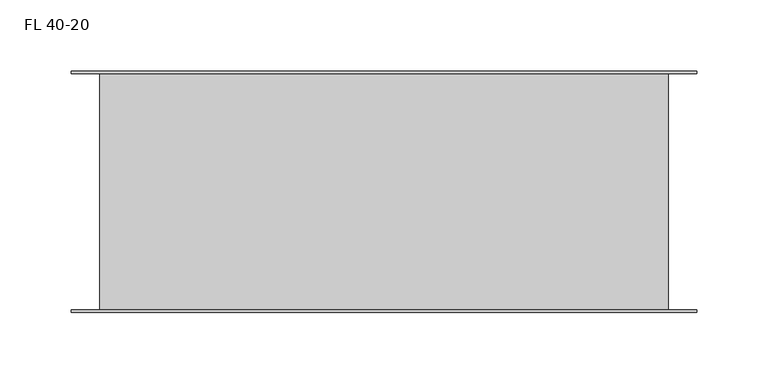
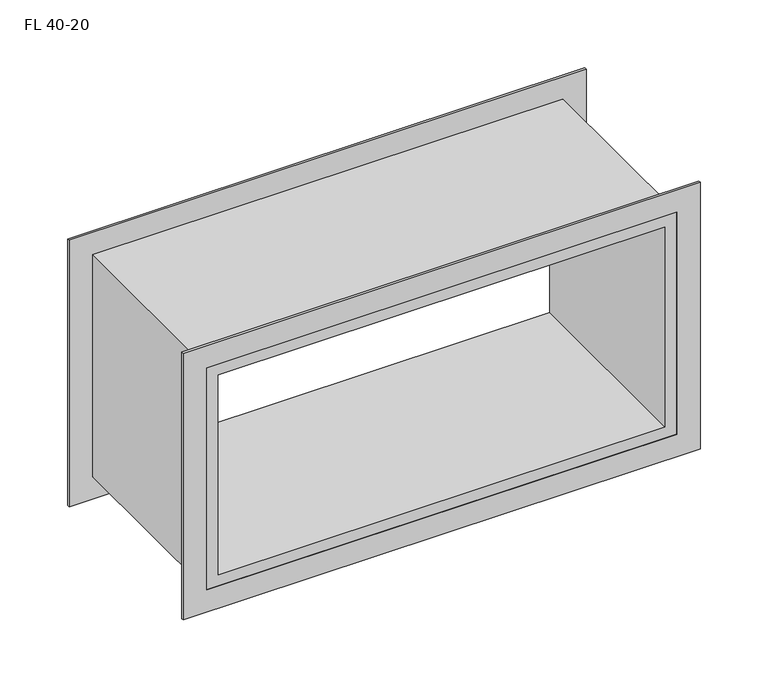
"""IFC4 building model written with IfcOpenShell, lengths in millimetres: proxy geometry, Обратный клапан FL : FL 40-20."""

from ifc_helpers import new_model, si_unit, frame, origin, place, context, project, spatial, polyline, outline, extrude, source, transform, mapped, element, save


def fl_40_20_b5c6f90e(model_context):
    return source(origin(), model_context, "Body", "SweptSolid", [
        extrude(outline(polyline([(120.0, 220.0), (120.0, -220.0), (-120.0, -220.0), (-120.0, 220.0), (120.0, 220.0)]), holes=[polyline([(-100.0, 200.0), (-100.0, -200.0), (100.0, -200.0), (100.0, 200.0), (-100.0, 200.0)])]), frame((0.0, 83.0, 0.0), z_axis=(0.0, 1.0, 0.0), x_axis=(0.0, 0.0, 1.0)), (0.0, 0.0, 1.0), 2.0),
        extrude(outline(polyline([(120.0, -220.0), (-120.0, -220.0), (-120.0, 220.0), (120.0, 220.0), (120.0, -220.0)]), holes=[polyline([(100.0, 200.0), (-100.0, 200.0), (-100.0, -200.0), (100.0, -200.0), (100.0, 200.0)])]), frame((0.0, -85.0, 0.0), z_axis=(0.0, 1.0, 0.0), x_axis=(0.0, 0.0, 1.0)), (0.0, 0.0, 1.0), 2.0),
        extrude(outline(polyline([(100.0, 200.0), (100.0, -200.0), (-100.0, -200.0), (-100.0, 200.0), (100.0, 200.0)]), holes=[polyline([(90.0, 190.0), (-90.0, 190.0), (-90.0, -190.0), (90.0, -190.0), (90.0, 190.0)])]), frame((0.0, -85.0, 0.0), z_axis=(0.0, 1.0, 0.0), x_axis=(0.0, 0.0, 1.0)), (0.0, 0.0, 1.0), 170.0),
    ])


if __name__ == "__main__":
    model = new_model("IFC4")
    model_context = context("Model", 3, world=origin())
    ifc_project = project(units=[si_unit("LENGTHUNIT", "METRE", prefix="MILLI")], contexts=[model_context])
    site = spatial("IfcSite", under=ifc_project)
    building = spatial("IfcBuilding", under=site)
    placement = place(None, origin())
    fl_40_20_shape = fl_40_20_b5c6f90e(model_context)
    element("IfcBuildingElementProxy", 1, Name="Обратный клапан FL : FL 40-20", ObjectType="Обратный клапан FL : FL 40-20", at=placement, inside=building, context=model_context, shape_type="MappedRepresentation", body=[
        mapped(fl_40_20_shape, transform((0.0, 0.0, 0.0), x_axis=(1.0, 0.0, 0.0), y_axis=(0.0, 1.0, 0.0), z_axis=(0.0, 0.0, 1.0))),
    ])
    save(model, "model.ifc")

# Revit data of these elements
# Type "Обратный клапан FL : FL 40-20"
#   Manufacturer = "WAER"
#   URL = "https://waer-air.com/"
#   ADSK_Система_Имя [instance default] = ""
#   ADSK_Наименование краткое = "FL 40-20"
#   ADSK_Наименование = "Обратный клапан FL 40-20"
#   ADSK_Масса_Текст = "4.4"
#   ADSK_Марка = ""
#   ADSK_Код изделия = ""
#   ADSK_Завод-изготовитель = "WAER"
#   ADSK_Единица измерения = "шт."
#   ADSK_Расход воздуха = 0 m³/h
#   ADSK_Размер_Ширина = 400 mm
#   ADSK_Размер_Высота = 200 mm
#   ADSK_Потеря давления воздуха = 0.0 Pa
#   ADSK_Масса = 4.4
#   ADSK_Количество = 1
#   Default Elevation = 0
#   Keynote = ""
